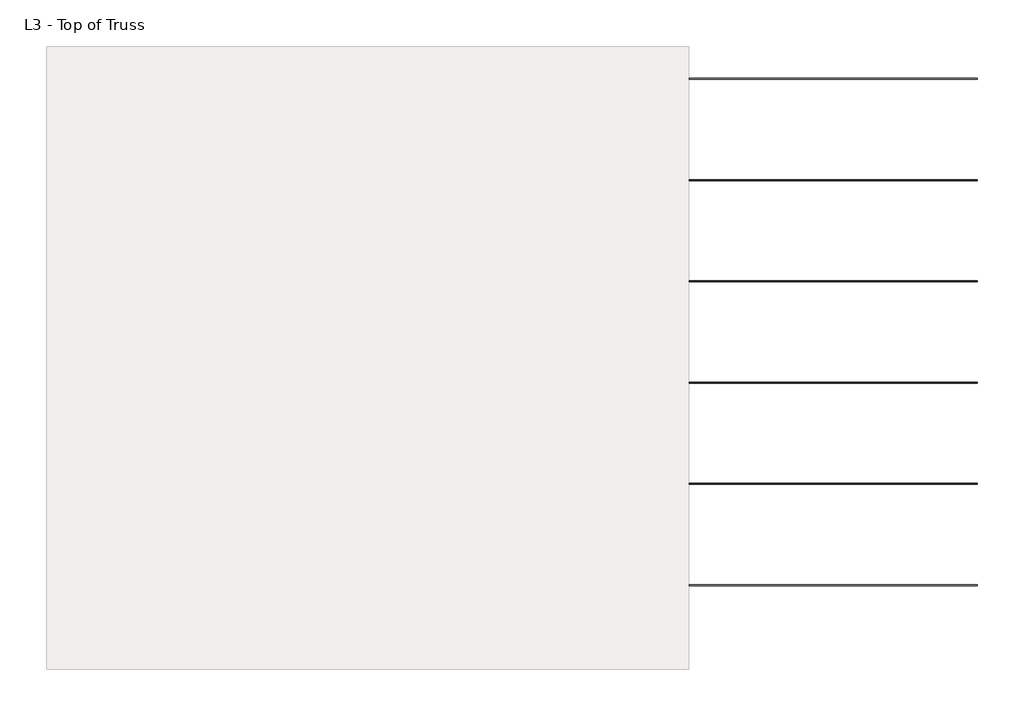
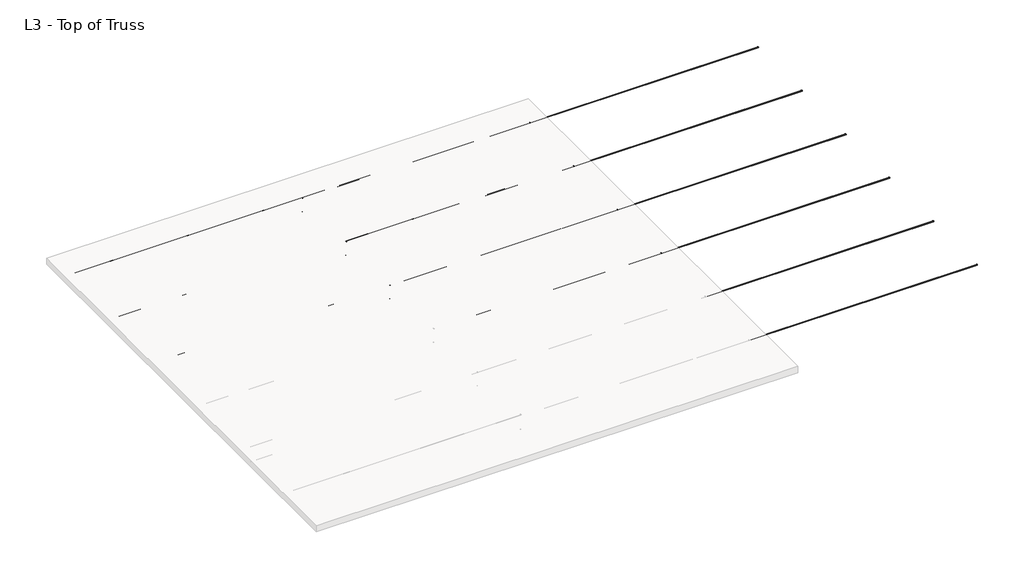
# One storey, part 2 of 2: 101 beams.
"""IFC4 building model written with IfcOpenShell, lengths in millimetres."""

import ifcopenshell
import ifcopenshell.guid

model = None  # the IFC model being written
_history = None  # IfcOwnerHistory: only IFC2X3 demands one
_inside = {}  # id of a spatial element -> (the spatial element, [elements in it])
_under = {}  # id of a project, library or spatial element -> (it, [spatial elements below it])
_declared = {}  # id of a project -> (the project, [libraries it declares])
_typed = {}  # id of a type object -> (the type object, [elements of that type])
_made_of = {}  # id of a material, layer set ... -> (it, [elements and type objects made of it])


def new_model(schema):
    """Start an empty IFC model of exactly this schema.

    Asked for "IFC4X3", IfcOpenShell would pick the latest addendum, in which some entities
    have other attributes; the version numbers below select the first issue.
    IFC2X3 requires an IfcOwnerHistory on every rooted entity: one is made here for all.
    """
    global model, _history
    if schema == "IFC4X3":
        model = ifcopenshell.file(schema_version=(4, 3, 0, 0))
    else:
        model = ifcopenshell.file(schema=schema)
    _inside.clear()
    _under.clear()
    _declared.clear()
    _typed.clear()
    _made_of.clear()
    _history = None
    if model.schema == "IFC2X3":
        org = make("IfcOrganization", Name="unknown")
        user = make(
            "IfcPersonAndOrganization",
            ThePerson=make("IfcPerson", FamilyName="unknown"),
            TheOrganization=org,
        )
        app = make(
            "IfcApplication",
            ApplicationDeveloper=org,
            Version="unknown",
            ApplicationFullName="unknown",
            ApplicationIdentifier="unknown",
        )
        _history = make(
            "IfcOwnerHistory",
            OwningUser=user,
            OwningApplication=app,
            ChangeAction="ADDED",
            CreationDate=0,
        )
    return model


def make(cls, **values):
    """One entity of the class cls with the attributes given. An attribute that is None is left unset."""
    return model.create_entity(
        cls, **{name: value for name, value in values.items() if value is not None}
    )


def rooted(cls, **values):
    """An entity with a GlobalId (a new one), such as an element, a storey or a relation."""
    return make(cls, GlobalId=ifcopenshell.guid.new(), OwnerHistory=_history, **values)


def si_unit(unit_type, name, prefix=None):
    """IfcSIUnit, for example si_unit("LENGTHUNIT", "METRE", prefix="MILLI")."""
    return make("IfcSIUnit", UnitType=unit_type, Prefix=prefix, Name=name)


def assignment(units):
    """IfcUnitAssignment: the units of a project."""
    return None if units is None else make("IfcUnitAssignment", Units=units)


def point(xyz):
    """IfcCartesianPoint."""
    return None if xyz is None else make("IfcCartesianPoint", Coordinates=xyz)


def direction(xyz):
    """IfcDirection."""
    return None if xyz is None else make("IfcDirection", DirectionRatios=xyz)


def frame(location, z_axis=None, x_axis=None):
    """IfcAxis2Placement3D, a coordinate frame: its origin and axes. An axis left out is left unset."""
    return make(
        "IfcAxis2Placement3D",
        Location=point(location),
        Axis=direction(z_axis),
        RefDirection=direction(x_axis),
    )


def frame_2d(location, x_axis=None):
    """IfcAxis2Placement2D, a coordinate frame in the plane: its origin and x axis."""
    return make(
        "IfcAxis2Placement2D", Location=point(location), RefDirection=direction(x_axis)
    )


def origin():
    """The frame at (0, 0, 0) with its axes left unset."""
    return frame((0.0, 0.0, 0.0))


def origin_2d():
    """The frame at (0, 0) in the plane with its x axis left unset."""
    return frame_2d((0.0, 0.0))


def place(relative_to, where):
    """IfcLocalPlacement: puts the frame where relative to a parent placement (None: the world)."""
    return make(
        "IfcLocalPlacement", PlacementRelTo=relative_to, RelativePlacement=where
    )


def context(
    kind, dimensions, precision=None, world=None, true_north=None, identifier=None
):
    """IfcGeometricRepresentationContext, for example the 3D "Model" context."""
    return make(
        "IfcGeometricRepresentationContext",
        ContextIdentifier=identifier,
        ContextType=kind,
        CoordinateSpaceDimension=dimensions,
        Precision=precision,
        WorldCoordinateSystem=world,
        TrueNorth=true_north,
    )


def project(units=None, contexts=None):
    """IfcProject with its units and contexts."""
    return rooted(
        "IfcProject",
        Name="project",
        RepresentationContexts=contexts,
        UnitsInContext=assignment(units),
    )


def spatial(cls, under=None, at=None, **own):
    """A site, building, storey or space (cls), placed at a placement, below another one or the project."""
    s = rooted(cls, ObjectPlacement=at, **own)
    if under is not None:
        _under.setdefault(under.id(), (under, []))[1].append(s)
    return s


def circle_curve(where, radius):
    """IfcCircle in the frame where."""
    return make("IfcCircle", Position=where, Radius=radius)


def trimmed(basis, trim1, trim2, sense, master):
    """IfcTrimmedCurve: the piece of a basis curve between two trims."""
    return make(
        "IfcTrimmedCurve",
        BasisCurve=basis,
        Trim1=trim1,
        Trim2=trim2,
        SenseAgreement=sense,
        MasterRepresentation=master,
    )


def segment(curve, same_sense, transition):
    """IfcCompositeCurveSegment."""
    return make(
        "IfcCompositeCurveSegment",
        Transition=transition,
        SameSense=same_sense,
        ParentCurve=curve,
    )


def composite_curve(segments, self_intersect=None):
    """IfcCompositeCurve: segments joined end to end."""
    return make("IfcCompositeCurve", Segments=segments, SelfIntersect=self_intersect)


def outline(outer, holes=None, kind="AREA"):
    """IfcArbitraryClosedProfileDef: a profile drawn as a closed curve; with holes, ...WithVoids."""
    if holes is None:
        return make("IfcArbitraryClosedProfileDef", ProfileType=kind, OuterCurve=outer)
    return make(
        "IfcArbitraryProfileDefWithVoids",
        ProfileType=kind,
        OuterCurve=outer,
        InnerCurves=holes,
    )


def extrude(swept, where, along, depth):
    """IfcExtrudedAreaSolid: the profile swept, set in the frame where, extruded along a direction by depth."""
    return make(
        "IfcExtrudedAreaSolid",
        SweptArea=swept,
        Position=where,
        ExtrudedDirection=direction(along),
        Depth=depth,
    )


def shape(context_of_items, identifier, shape_type, items):
    """IfcShapeRepresentation: the items that make up one representation, for example the "Body"."""
    return make(
        "IfcShapeRepresentation",
        ContextOfItems=context_of_items,
        RepresentationIdentifier=identifier,
        RepresentationType=shape_type,
        Items=items,
    )


def source(mapping_origin, context_of_items, identifier, shape_type, items):
    """IfcRepresentationMap: a shape defined once, which mapped items show again and again."""
    return make(
        "IfcRepresentationMap",
        MappingOrigin=mapping_origin,
        MappedRepresentation=shape(context_of_items, identifier, shape_type, items),
    )


def transform(
    local_origin,
    x_axis=None,
    y_axis=None,
    z_axis=None,
    scale=None,
    scale2=None,
    scale3=None,
    uniform=True,
):
    """IfcCartesianTransformationOperator3D, or its non-uniform kind. x_axis, y_axis, z_axis: its Axis1, 2, 3."""
    if uniform:
        return make(
            "IfcCartesianTransformationOperator3D",
            Axis1=direction(x_axis),
            Axis2=direction(y_axis),
            LocalOrigin=point(local_origin),
            Scale=scale,
            Axis3=direction(z_axis),
        )
    return make(
        "IfcCartesianTransformationOperator3DnonUniform",
        Axis1=direction(x_axis),
        Axis2=direction(y_axis),
        LocalOrigin=point(local_origin),
        Scale=scale,
        Axis3=direction(z_axis),
        Scale2=scale2,
        Scale3=scale3,
    )


def mapped(mapping_source, mapping_target):
    """IfcMappedItem: shows the shape of a source again, moved by a transform."""
    return make(
        "IfcMappedItem", MappingSource=mapping_source, MappingTarget=mapping_target
    )


def made_of(thing, what):
    """Note that an element or type object is made of a material, layer set ...; save() writes the relation."""
    if what is not None:
        _made_of.setdefault(what.id(), (what, []))[1].append(thing)
    return thing


def element(
    cls,
    number,
    at=None,
    inside=None,
    cuts=None,
    type_object=None,
    material=None,
    context=None,
    identifier="Body",
    shape_type=None,
    held_by="IfcProductDefinitionShape",
    body=None,
    shapes=None,
    **own,
):
    """One element of the class cls, such as IfcWall. Its Tag is "e" and its number.

    at: its placement. inside: the storey or other place that contains it. cuts: it is an
    opening in that element (IfcRelVoidsElement). A single representation is given by context,
    identifier, shape_type and body (its items); several are given by shapes. held_by: the class
    of the entity that holds the representations. save() writes the other relations.
    """
    e = rooted(cls, Tag="e%d" % number, ObjectPlacement=at, **own)
    if body is not None:
        shapes = [shape(context, identifier, shape_type, body)]
    if shapes is not None:
        e.Representation = make(held_by, Representations=shapes)
    if inside is not None:
        _inside.setdefault(inside.id(), (inside, []))[1].append(e)
    if cuts is not None:
        rooted(
            "IfcRelVoidsElement", RelatingBuildingElement=cuts, RelatedOpeningElement=e
        )
    if type_object is not None:
        _typed.setdefault(type_object.id(), (type_object, []))[1].append(e)
    return made_of(e, material)


def aggregate(whole, parts):
    """IfcRelAggregates: a whole, such as a stair, and the parts it consists of."""
    return rooted("IfcRelAggregates", RelatingObject=whole, RelatedObjects=parts)


def save(model, path):
    """Write the relations noted so far, then the file.

    IfcRelAggregates (storeys below a building ...), IfcRelContainedInSpatialStructure (elements
    in a storey), IfcRelDefinesByType, IfcRelAssociatesMaterial and IfcRelDeclares: one each for
    every whole, place, type object, material and project.
    """
    for whole, parts in _under.values():
        aggregate(whole, parts)
    for where, things in _inside.values():
        rooted(
            "IfcRelContainedInSpatialStructure",
            RelatedElements=things,
            RelatingStructure=where,
        )
    for kind, things in _typed.values():
        rooted("IfcRelDefinesByType", RelatedObjects=things, RelatingType=kind)
    for what, things in _made_of.values():
        rooted("IfcRelAssociatesMaterial", RelatedObjects=things, RelatingMaterial=what)
    for by, libraries in _declared.values():
        rooted("IfcRelDeclares", RelatingContext=by, RelatedDefinitions=libraries)
    model.write(path)


def circular_hollow_sections_chs60_3x5_c94bd862(model_context):
    return source(origin(), model_context, "Body", "SweptSolid", [
        extrude(outline(composite_curve([segment(trimmed(circle_curve(origin_2d(), 30.15), [point((-30.15, 0.0))], [point((30.15, 0.0))], False, "CARTESIAN"), True, "CONTINUOUS"), segment(trimmed(circle_curve(origin_2d(), 30.15), [point((30.15, 0.0))], [point((-30.15, 0.0))], False, "CARTESIAN"), True, "CONTINUOUS")], self_intersect=False), holes=[composite_curve([segment(trimmed(circle_curve(origin_2d(), 25.15), [point((25.15, 0.0))], [point((-25.15, 0.0))], True, "CARTESIAN"), True, "CONTINUOUS"), segment(trimmed(circle_curve(origin_2d(), 25.15), [point((-25.15, 0.0))], [point((25.15, 0.0))], True, "CARTESIAN"), True, "CONTINUOUS")], self_intersect=False)]), frame((-557.0, 0.0, 0.0), z_axis=(1.0, 0.0, 0.0), x_axis=(0.0, 1.0, 0.0)), (0.0, 0.0, 1.0), 1114.0),
    ])


def circular_hollow_sections_chs60_3x5_b8a643cb(model_context):
    return source(origin(), model_context, "Body", "SweptSolid", [
        extrude(outline(composite_curve([segment(trimmed(circle_curve(origin_2d(), 30.15), [point((-30.15, 0.0))], [point((30.15, 0.0))], False, "CARTESIAN"), True, "CONTINUOUS"), segment(trimmed(circle_curve(origin_2d(), 30.15), [point((30.15, 0.0))], [point((-30.15, 0.0))], False, "CARTESIAN"), True, "CONTINUOUS")], self_intersect=False), holes=[composite_curve([segment(trimmed(circle_curve(origin_2d(), 25.15), [point((25.15, 0.0))], [point((-25.15, 0.0))], True, "CARTESIAN"), True, "CONTINUOUS"), segment(trimmed(circle_curve(origin_2d(), 25.15), [point((-25.15, 0.0))], [point((25.15, 0.0))], True, "CARTESIAN"), True, "CONTINUOUS")], self_intersect=False)]), frame((-790.0, 0.0, 0.0), z_axis=(1.0, 0.0, 0.0), x_axis=(0.0, 1.0, 0.0)), (0.0, 0.0, 1.0), 1580.0),
    ])


def circular_hollow_sections_chs60_3x5_ee2473de(model_context):
    return source(origin(), model_context, "Body", "SweptSolid", [
        extrude(outline(composite_curve([segment(trimmed(circle_curve(origin_2d(), 30.15), [point((-30.15, 0.0))], [point((30.15, 0.0))], False, "CARTESIAN"), True, "CONTINUOUS"), segment(trimmed(circle_curve(origin_2d(), 30.15), [point((30.15, 0.0))], [point((-30.15, 0.0))], False, "CARTESIAN"), True, "CONTINUOUS")], self_intersect=False), holes=[composite_curve([segment(trimmed(circle_curve(origin_2d(), 25.15), [point((25.15, 0.0))], [point((-25.15, 0.0))], True, "CARTESIAN"), True, "CONTINUOUS"), segment(trimmed(circle_curve(origin_2d(), 25.15), [point((-25.15, 0.0))], [point((25.15, 0.0))], True, "CARTESIAN"), True, "CONTINUOUS")], self_intersect=False)]), frame((-9000.0, 0.0, 0.0), z_axis=(1.0, 0.0, 0.0), x_axis=(0.0, 1.0, 0.0)), (0.0, 0.0, 1.0), 18000.0),
    ])


def circular_hollow_sections_chs60_3x5_7809bf4e(model_context):
    return source(origin(), model_context, "Body", "SweptSolid", [
        extrude(outline(composite_curve([segment(trimmed(circle_curve(origin_2d(), 30.15), [point((-30.15, 0.0))], [point((30.15, 0.0))], False, "CARTESIAN"), True, "CONTINUOUS"), segment(trimmed(circle_curve(origin_2d(), 30.15), [point((30.15, 0.0))], [point((-30.15, 0.0))], False, "CARTESIAN"), True, "CONTINUOUS")], self_intersect=False), holes=[composite_curve([segment(trimmed(circle_curve(origin_2d(), 25.15), [point((25.15, 0.0))], [point((-25.15, 0.0))], True, "CARTESIAN"), True, "CONTINUOUS"), segment(trimmed(circle_curve(origin_2d(), 25.15), [point((-25.15, 0.0))], [point((25.15, 0.0))], True, "CARTESIAN"), True, "CONTINUOUS")], self_intersect=False)]), frame((-600.0, 0.0, 0.0), z_axis=(1.0, 0.0, 0.0), x_axis=(0.0, 1.0, 0.0)), (0.0, 0.0, 1.0), 1157.0),
    ])


model = new_model("IFC4")

# Units and contexts
model_context = context("Model", 3, world=origin())
ifc_project = project(units=[si_unit("LENGTHUNIT", "METRE", prefix="MILLI")], contexts=[model_context])

# Site, building, storey
site = spatial("IfcSite", under=ifc_project)
building = spatial("IfcBuilding", under=site)
storey = spatial("IfcBuildingStorey", under=building, Name="L3 - Top of Truss", Elevation=7800.0)

# Beams
placement = place(None, origin())
circular_hollow_sections_chs60_3x5_shape = circular_hollow_sections_chs60_3x5_c94bd862(model_context)
element("IfcBeam", 1, ObjectType="Circular Hollow Sections : CHS60.3x5", at=placement, inside=storey, context=model_context, shape_type="MappedRepresentation", body=[
    mapped(circular_hollow_sections_chs60_3x5_shape, transform((9574.7303686, 941.2380918, 7200.0), x_axis=(0.0, 0.0, 1.0), y_axis=(0.0, -1.0, 0.0), z_axis=(1.0, 0.0, 0.0))),
])
element("IfcBeam", 2, ObjectType="Circular Hollow Sections : CHS60.3x5", at=placement, inside=storey, context=model_context, shape_type="MappedRepresentation", body=[
    mapped(circular_hollow_sections_chs60_3x5_shape, transform((-5853.84106, 941.2380918, 7200.0), x_axis=(0.0, 0.0, 1.0), y_axis=(0.0, -1.0, 0.0), z_axis=(1.0, 0.0, 0.0))),
])
element("IfcBeam", 3, ObjectType="Circular Hollow Sections : CHS60.3x5", at=placement, inside=storey, context=model_context, shape_type="MappedRepresentation", body=[
    mapped(circular_hollow_sections_chs60_3x5_shape, transform((8289.0160829, 941.2380918, 7200.0), x_axis=(0.0, 0.0, 1.0), y_axis=(0.0, -1.0, 0.0), z_axis=(1.0, 0.0, 0.0))),
])
element("IfcBeam", 4, ObjectType="Circular Hollow Sections : CHS60.3x5", at=placement, inside=storey, context=model_context, shape_type="MappedRepresentation", body=[
    mapped(circular_hollow_sections_chs60_3x5_shape, transform((-4568.1267743, 941.2380918, 7200.0), x_axis=(0.0, 0.0, 1.0), y_axis=(0.0, -1.0, 0.0), z_axis=(1.0, 0.0, 0.0))),
])
element("IfcBeam", 5, ObjectType="Circular Hollow Sections : CHS60.3x5", at=placement, inside=storey, context=model_context, shape_type="MappedRepresentation", body=[
    mapped(circular_hollow_sections_chs60_3x5_shape, transform((7003.3017972, 941.2380918, 7200.0), x_axis=(0.0, 0.0, 1.0), y_axis=(0.0, -1.0, 0.0), z_axis=(1.0, 0.0, 0.0))),
])
element("IfcBeam", 6, ObjectType="Circular Hollow Sections : CHS60.3x5", at=placement, inside=storey, context=model_context, shape_type="MappedRepresentation", body=[
    mapped(circular_hollow_sections_chs60_3x5_shape, transform((-3282.4124885, 941.2380918, 7200.0), x_axis=(0.0, 0.0, 1.0), y_axis=(0.0, -1.0, 0.0), z_axis=(1.0, 0.0, 0.0))),
])
element("IfcBeam", 7, ObjectType="Circular Hollow Sections : CHS60.3x5", at=placement, inside=storey, context=model_context, shape_type="MappedRepresentation", body=[
    mapped(circular_hollow_sections_chs60_3x5_shape, transform((5717.5875115, 941.2380918, 7200.0), x_axis=(0.0, 0.0, 1.0), y_axis=(0.0, -1.0, 0.0), z_axis=(1.0, 0.0, 0.0))),
])
element("IfcBeam", 8, ObjectType="Circular Hollow Sections : CHS60.3x5", at=placement, inside=storey, context=model_context, shape_type="MappedRepresentation", body=[
    mapped(circular_hollow_sections_chs60_3x5_shape, transform((4431.8732257, 941.2380918, 7200.0), x_axis=(0.0, 0.0, 1.0), y_axis=(0.0, -1.0, 0.0), z_axis=(1.0, 0.0, 0.0))),
])
element("IfcBeam", 9, ObjectType="Circular Hollow Sections : CHS60.3x5", at=placement, inside=storey, context=model_context, shape_type="MappedRepresentation", body=[
    mapped(circular_hollow_sections_chs60_3x5_shape, transform((3146.15894, 941.2380918, 7200.0), x_axis=(0.0, 0.0, 1.0), y_axis=(0.0, -1.0, 0.0), z_axis=(1.0, 0.0, 0.0))),
])
element("IfcBeam", 10, ObjectType="Circular Hollow Sections : CHS60.3x5", at=placement, inside=storey, context=model_context, shape_type="MappedRepresentation", body=[
    mapped(circular_hollow_sections_chs60_3x5_shape, transform((-1996.6982028, 941.2380918, 7200.0), x_axis=(0.0, 0.0, 1.0), y_axis=(0.0, -1.0, 0.0), z_axis=(1.0, 0.0, 0.0))),
])
element("IfcBeam", 11, ObjectType="Circular Hollow Sections : CHS60.3x5", at=placement, inside=storey, context=model_context, shape_type="MappedRepresentation", body=[
    mapped(circular_hollow_sections_chs60_3x5_shape, transform((-710.9839171, 941.2380918, 7200.0), x_axis=(0.0, 0.0, 1.0), y_axis=(0.0, -1.0, 0.0), z_axis=(1.0, 0.0, 0.0))),
])
element("IfcBeam", 12, ObjectType="Circular Hollow Sections : CHS60.3x5", at=placement, inside=storey, context=model_context, shape_type="MappedRepresentation", body=[
    mapped(circular_hollow_sections_chs60_3x5_shape, transform((574.7303686, 941.2380918, 7200.0), x_axis=(0.0, 0.0, 1.0), y_axis=(0.0, -1.0, 0.0), z_axis=(1.0, 0.0, 0.0))),
])
element("IfcBeam", 13, ObjectType="Circular Hollow Sections : CHS60.3x5", at=placement, inside=storey, context=model_context, shape_type="MappedRepresentation", body=[
    mapped(circular_hollow_sections_chs60_3x5_shape, transform((1860.4446543, 941.2380918, 7200.0), x_axis=(0.0, 0.0, 1.0), y_axis=(0.0, -1.0, 0.0), z_axis=(1.0, 0.0, 0.0))),
])
element("IfcBeam", 14, ObjectType="Circular Hollow Sections : CHS60.3x5", at=placement, inside=storey, context=model_context, shape_type="MappedRepresentation", body=[
    mapped(circular_hollow_sections_chs60_3x5_shape, transform((9574.7303686, 6941.2380918, 7200.0), x_axis=(0.0, 0.0, 1.0), y_axis=(0.0, -1.0, 0.0), z_axis=(1.0, 0.0, 0.0))),
])
element("IfcBeam", 15, ObjectType="Circular Hollow Sections : CHS60.3x5", at=placement, inside=storey, context=model_context, shape_type="MappedRepresentation", body=[
    mapped(circular_hollow_sections_chs60_3x5_shape, transform((-5853.84106, 6941.2380918, 7200.0), x_axis=(0.0, 0.0, 1.0), y_axis=(0.0, -1.0, 0.0), z_axis=(1.0, 0.0, 0.0))),
])
element("IfcBeam", 16, ObjectType="Circular Hollow Sections : CHS60.3x5", at=placement, inside=storey, context=model_context, shape_type="MappedRepresentation", body=[
    mapped(circular_hollow_sections_chs60_3x5_shape, transform((8289.0160829, 6941.2380918, 7200.0), x_axis=(0.0, 0.0, 1.0), y_axis=(0.0, -1.0, 0.0), z_axis=(1.0, 0.0, 0.0))),
])
element("IfcBeam", 17, ObjectType="Circular Hollow Sections : CHS60.3x5", at=placement, inside=storey, context=model_context, shape_type="MappedRepresentation", body=[
    mapped(circular_hollow_sections_chs60_3x5_shape, transform((-4568.1267743, 6941.2380918, 7200.0), x_axis=(0.0, 0.0, 1.0), y_axis=(0.0, -1.0, 0.0), z_axis=(1.0, 0.0, 0.0))),
])
element("IfcBeam", 18, ObjectType="Circular Hollow Sections : CHS60.3x5", at=placement, inside=storey, context=model_context, shape_type="MappedRepresentation", body=[
    mapped(circular_hollow_sections_chs60_3x5_shape, transform((7003.3017972, 6941.2380918, 7200.0), x_axis=(0.0, 0.0, 1.0), y_axis=(0.0, -1.0, 0.0), z_axis=(1.0, 0.0, 0.0))),
])
element("IfcBeam", 19, ObjectType="Circular Hollow Sections : CHS60.3x5", at=placement, inside=storey, context=model_context, shape_type="MappedRepresentation", body=[
    mapped(circular_hollow_sections_chs60_3x5_shape, transform((-3282.4124885, 6941.2380918, 7200.0), x_axis=(0.0, 0.0, 1.0), y_axis=(0.0, -1.0, 0.0), z_axis=(1.0, 0.0, 0.0))),
])
element("IfcBeam", 20, ObjectType="Circular Hollow Sections : CHS60.3x5", at=placement, inside=storey, context=model_context, shape_type="MappedRepresentation", body=[
    mapped(circular_hollow_sections_chs60_3x5_shape, transform((5717.5875115, 6941.2380918, 7200.0), x_axis=(0.0, 0.0, 1.0), y_axis=(0.0, -1.0, 0.0), z_axis=(1.0, 0.0, 0.0))),
])
element("IfcBeam", 21, ObjectType="Circular Hollow Sections : CHS60.3x5", at=placement, inside=storey, context=model_context, shape_type="MappedRepresentation", body=[
    mapped(circular_hollow_sections_chs60_3x5_shape, transform((4431.8732257, 6941.2380918, 7200.0), x_axis=(0.0, 0.0, 1.0), y_axis=(0.0, -1.0, 0.0), z_axis=(1.0, 0.0, 0.0))),
])
element("IfcBeam", 22, ObjectType="Circular Hollow Sections : CHS60.3x5", at=placement, inside=storey, context=model_context, shape_type="MappedRepresentation", body=[
    mapped(circular_hollow_sections_chs60_3x5_shape, transform((3146.15894, 6941.2380918, 7200.0), x_axis=(0.0, 0.0, 1.0), y_axis=(0.0, -1.0, 0.0), z_axis=(1.0, 0.0, 0.0))),
])
element("IfcBeam", 23, ObjectType="Circular Hollow Sections : CHS60.3x5", at=placement, inside=storey, context=model_context, shape_type="MappedRepresentation", body=[
    mapped(circular_hollow_sections_chs60_3x5_shape, transform((-1996.6982028, 6941.2380918, 7200.0), x_axis=(0.0, 0.0, 1.0), y_axis=(0.0, -1.0, 0.0), z_axis=(1.0, 0.0, 0.0))),
])
element("IfcBeam", 24, ObjectType="Circular Hollow Sections : CHS60.3x5", at=placement, inside=storey, context=model_context, shape_type="MappedRepresentation", body=[
    mapped(circular_hollow_sections_chs60_3x5_shape, transform((-710.9839171, 6941.2380918, 7200.0), x_axis=(0.0, 0.0, 1.0), y_axis=(0.0, -1.0, 0.0), z_axis=(1.0, 0.0, 0.0))),
])
element("IfcBeam", 25, ObjectType="Circular Hollow Sections : CHS60.3x5", at=placement, inside=storey, context=model_context, shape_type="MappedRepresentation", body=[
    mapped(circular_hollow_sections_chs60_3x5_shape, transform((574.7303686, 6941.2380918, 7200.0), x_axis=(0.0, 0.0, 1.0), y_axis=(0.0, -1.0, 0.0), z_axis=(1.0, 0.0, 0.0))),
])
element("IfcBeam", 26, ObjectType="Circular Hollow Sections : CHS60.3x5", at=placement, inside=storey, context=model_context, shape_type="MappedRepresentation", body=[
    mapped(circular_hollow_sections_chs60_3x5_shape, transform((1860.4446543, 6941.2380918, 7200.0), x_axis=(0.0, 0.0, 1.0), y_axis=(0.0, -1.0, 0.0), z_axis=(1.0, 0.0, 0.0))),
])
element("IfcBeam", 27, ObjectType="Circular Hollow Sections : CHS60.3x5", at=placement, inside=storey, context=model_context, shape_type="MappedRepresentation", body=[
    mapped(circular_hollow_sections_chs60_3x5_shape, transform((9574.7303686, -5058.7619082, 7200.0), x_axis=(0.0, 0.0, 1.0), y_axis=(0.0, -1.0, 0.0), z_axis=(1.0, 0.0, 0.0))),
])
element("IfcBeam", 28, ObjectType="Circular Hollow Sections : CHS60.3x5", at=placement, inside=storey, context=model_context, shape_type="MappedRepresentation", body=[
    mapped(circular_hollow_sections_chs60_3x5_shape, transform((8289.0160829, -5058.7619082, 7200.0), x_axis=(0.0, 0.0, 1.0), y_axis=(0.0, -1.0, 0.0), z_axis=(1.0, 0.0, 0.0))),
])
element("IfcBeam", 29, ObjectType="Circular Hollow Sections : CHS60.3x5", at=placement, inside=storey, context=model_context, shape_type="MappedRepresentation", body=[
    mapped(circular_hollow_sections_chs60_3x5_shape, transform((7003.3017972, -5058.7619082, 7200.0), x_axis=(0.0, 0.0, 1.0), y_axis=(0.0, -1.0, 0.0), z_axis=(1.0, 0.0, 0.0))),
])
element("IfcBeam", 30, ObjectType="Circular Hollow Sections : CHS60.3x5", at=placement, inside=storey, context=model_context, shape_type="MappedRepresentation", body=[
    mapped(circular_hollow_sections_chs60_3x5_shape, transform((5717.5875115, -5058.7619082, 7200.0), x_axis=(0.0, 0.0, 1.0), y_axis=(0.0, -1.0, 0.0), z_axis=(1.0, 0.0, 0.0))),
])
element("IfcBeam", 31, ObjectType="Circular Hollow Sections : CHS60.3x5", at=placement, inside=storey, context=model_context, shape_type="MappedRepresentation", body=[
    mapped(circular_hollow_sections_chs60_3x5_shape, transform((4431.8732257, -5058.7619082, 7200.0), x_axis=(0.0, 0.0, 1.0), y_axis=(0.0, -1.0, 0.0), z_axis=(1.0, 0.0, 0.0))),
])
element("IfcBeam", 32, ObjectType="Circular Hollow Sections : CHS60.3x5", at=placement, inside=storey, context=model_context, shape_type="MappedRepresentation", body=[
    mapped(circular_hollow_sections_chs60_3x5_shape, transform((3146.15894, -5058.7619082, 7200.0), x_axis=(0.0, 0.0, 1.0), y_axis=(0.0, -1.0, 0.0), z_axis=(1.0, 0.0, 0.0))),
])
element("IfcBeam", 33, ObjectType="Circular Hollow Sections : CHS60.3x5", at=placement, inside=storey, context=model_context, shape_type="MappedRepresentation", body=[
    mapped(circular_hollow_sections_chs60_3x5_shape, transform((574.7303686, -5058.7619082, 7200.0), x_axis=(0.0, 0.0, 1.0), y_axis=(0.0, -1.0, 0.0), z_axis=(1.0, 0.0, 0.0))),
])
element("IfcBeam", 34, ObjectType="Circular Hollow Sections : CHS60.3x5", at=placement, inside=storey, context=model_context, shape_type="MappedRepresentation", body=[
    mapped(circular_hollow_sections_chs60_3x5_shape, transform((1860.4446543, -5058.7619082, 7200.0), x_axis=(0.0, 0.0, 1.0), y_axis=(0.0, -1.0, 0.0), z_axis=(1.0, 0.0, 0.0))),
])
element("IfcBeam", 35, ObjectType="Circular Hollow Sections : CHS60.3x5", at=placement, inside=storey, context=model_context, shape_type="MappedRepresentation", body=[
    mapped(circular_hollow_sections_chs60_3x5_shape, transform((9574.7303686, -11058.7619082, 7200.0), x_axis=(0.0, 0.0, 1.0), y_axis=(0.0, -1.0, 0.0), z_axis=(1.0, 0.0, 0.0))),
])
element("IfcBeam", 36, ObjectType="Circular Hollow Sections : CHS60.3x5", at=placement, inside=storey, context=model_context, shape_type="MappedRepresentation", body=[
    mapped(circular_hollow_sections_chs60_3x5_shape, transform((8289.0160829, -11058.7619082, 7200.0), x_axis=(0.0, 0.0, 1.0), y_axis=(0.0, -1.0, 0.0), z_axis=(1.0, 0.0, 0.0))),
])
element("IfcBeam", 37, ObjectType="Circular Hollow Sections : CHS60.3x5", at=placement, inside=storey, context=model_context, shape_type="MappedRepresentation", body=[
    mapped(circular_hollow_sections_chs60_3x5_shape, transform((7003.3017972, -11058.7619082, 7200.0), x_axis=(0.0, 0.0, 1.0), y_axis=(0.0, -1.0, 0.0), z_axis=(1.0, 0.0, 0.0))),
])
circular_hollow_sections_chs60_3x5_2_shape = circular_hollow_sections_chs60_3x5_b8a643cb(model_context)
element("IfcBeam", 38, ObjectType="Circular Hollow Sections : CHS60.3x5", at=placement, inside=storey, context=model_context, shape_type="MappedRepresentation", body=[
    mapped(circular_hollow_sections_chs60_3x5_2_shape, transform((8931.8732257, 941.2380918, 7200.0), x_axis=(0.7310552682428691, 0.0, 0.6823182503600111), y_axis=(0.0, -1.0, 0.0), z_axis=(0.6823182503600111, 0.0, -0.7310552682428691))),
])
element("IfcBeam", 39, ObjectType="Circular Hollow Sections : CHS60.3x5", at=placement, inside=storey, context=model_context, shape_type="MappedRepresentation", body=[
    mapped(circular_hollow_sections_chs60_3x5_2_shape, transform((-5210.9839171, 941.2380918, 7200.0), x_axis=(0.7310552682428689, 0.0, -0.6823182503600113), y_axis=(0.0, -1.0, 0.0), z_axis=(-0.6823182503600113, 0.0, -0.7310552682428689))),
])
element("IfcBeam", 40, ObjectType="Circular Hollow Sections : CHS60.3x5", at=placement, inside=storey, context=model_context, shape_type="MappedRepresentation", body=[
    mapped(circular_hollow_sections_chs60_3x5_2_shape, transform((7646.15894, 941.2380918, 7200.0), x_axis=(0.7310552682428691, 0.0, 0.6823182503600111), y_axis=(0.0, -1.0, 0.0), z_axis=(0.6823182503600111, 0.0, -0.7310552682428691))),
])
element("IfcBeam", 41, ObjectType="Circular Hollow Sections : CHS60.3x5", at=placement, inside=storey, context=model_context, shape_type="MappedRepresentation", body=[
    mapped(circular_hollow_sections_chs60_3x5_2_shape, transform((-3925.2696314, 941.2380918, 7200.0), x_axis=(0.7310552682428689, 0.0, -0.6823182503600113), y_axis=(0.0, -1.0, 0.0), z_axis=(-0.6823182503600113, 0.0, -0.7310552682428689))),
])
element("IfcBeam", 42, ObjectType="Circular Hollow Sections : CHS60.3x5", at=placement, inside=storey, context=model_context, shape_type="MappedRepresentation", body=[
    mapped(circular_hollow_sections_chs60_3x5_2_shape, transform((6360.4446543, 941.2380918, 7200.0), x_axis=(0.7310552682428691, 0.0, 0.6823182503600111), y_axis=(0.0, -1.0, 0.0), z_axis=(0.6823182503600111, 0.0, -0.7310552682428691))),
])
element("IfcBeam", 43, ObjectType="Circular Hollow Sections : CHS60.3x5", at=placement, inside=storey, context=model_context, shape_type="MappedRepresentation", body=[
    mapped(circular_hollow_sections_chs60_3x5_2_shape, transform((-2639.5553457, 941.2380918, 7200.0), x_axis=(0.7310552682428689, 0.0, -0.6823182503600113), y_axis=(0.0, -1.0, 0.0), z_axis=(-0.6823182503600113, 0.0, -0.7310552682428689))),
])
element("IfcBeam", 44, ObjectType="Circular Hollow Sections : CHS60.3x5", at=placement, inside=storey, context=model_context, shape_type="MappedRepresentation", body=[
    mapped(circular_hollow_sections_chs60_3x5_2_shape, transform((5074.7303686, 941.2380918, 7200.0), x_axis=(0.7310552682428691, 0.0, 0.6823182503600111), y_axis=(0.0, -1.0, 0.0), z_axis=(0.6823182503600111, 0.0, -0.7310552682428691))),
])
element("IfcBeam", 45, ObjectType="Circular Hollow Sections : CHS60.3x5", at=placement, inside=storey, context=model_context, shape_type="MappedRepresentation", body=[
    mapped(circular_hollow_sections_chs60_3x5_2_shape, transform((3789.0160829, 941.2380918, 7200.0), x_axis=(0.7310552682428691, 0.0, 0.6823182503600111), y_axis=(0.0, -1.0, 0.0), z_axis=(0.6823182503600111, 0.0, -0.7310552682428691))),
])
element("IfcBeam", 46, ObjectType="Circular Hollow Sections : CHS60.3x5", at=placement, inside=storey, context=model_context, shape_type="MappedRepresentation", body=[
    mapped(circular_hollow_sections_chs60_3x5_2_shape, transform((10217.5875115, 941.2380918, 7200.0), x_axis=(0.7310552682428691, 0.0, 0.6823182503600111), y_axis=(0.0, -1.0, 0.0), z_axis=(0.6823182503600111, 0.0, -0.7310552682428691))),
])
element("IfcBeam", 47, ObjectType="Circular Hollow Sections : CHS60.3x5", at=placement, inside=storey, context=model_context, shape_type="MappedRepresentation", body=[
    mapped(circular_hollow_sections_chs60_3x5_2_shape, transform((2503.3017972, 941.2380918, 7200.0), x_axis=(0.7310552682428691, 0.0, 0.682318250360011), y_axis=(0.0, -1.0, 0.0), z_axis=(0.682318250360011, 0.0, -0.7310552682428691))),
])
element("IfcBeam", 48, ObjectType="Circular Hollow Sections : CHS60.3x5", at=placement, inside=storey, context=model_context, shape_type="MappedRepresentation", body=[
    mapped(circular_hollow_sections_chs60_3x5_2_shape, transform((-1353.84106, 941.2380918, 7200.0), x_axis=(0.7310552682428689, 0.0, -0.6823182503600113), y_axis=(0.0, -1.0, 0.0), z_axis=(-0.6823182503600113, 0.0, -0.7310552682428689))),
])
element("IfcBeam", 49, ObjectType="Circular Hollow Sections : CHS60.3x5", at=placement, inside=storey, context=model_context, shape_type="MappedRepresentation", body=[
    mapped(circular_hollow_sections_chs60_3x5_2_shape, transform((-68.1267743, 941.2380918, 7200.0), x_axis=(0.7310552682428689, 0.0, -0.6823182503600113), y_axis=(0.0, -1.0, 0.0), z_axis=(-0.6823182503600113, 0.0, -0.7310552682428689))),
])
element("IfcBeam", 50, ObjectType="Circular Hollow Sections : CHS60.3x5", at=placement, inside=storey, context=model_context, shape_type="MappedRepresentation", body=[
    mapped(circular_hollow_sections_chs60_3x5_2_shape, transform((-6496.6982028, 941.2380918, 7200.0), x_axis=(0.7310552682428688, 0.0, -0.6823182503600115), y_axis=(0.0, -1.0, 0.0), z_axis=(-0.6823182503600115, 0.0, -0.7310552682428688))),
])
element("IfcBeam", 51, ObjectType="Circular Hollow Sections : CHS60.3x5", at=placement, inside=storey, context=model_context, shape_type="MappedRepresentation", body=[
    mapped(circular_hollow_sections_chs60_3x5_2_shape, transform((1217.5875115, 941.2380918, 7200.0), x_axis=(0.7310552682428689, 0.0, -0.6823182503600113), y_axis=(0.0, -1.0, 0.0), z_axis=(-0.6823182503600113, 0.0, -0.7310552682428689))),
])
element("IfcBeam", 52, ObjectType="Circular Hollow Sections : CHS60.3x5", at=placement, inside=storey, context=model_context, shape_type="MappedRepresentation", body=[
    mapped(circular_hollow_sections_chs60_3x5_2_shape, transform((8931.8732257, 6941.2380918, 7200.0), x_axis=(0.7310552682428691, 0.0, 0.6823182503600111), y_axis=(0.0, -1.0, 0.0), z_axis=(0.6823182503600111, 0.0, -0.7310552682428691))),
])
element("IfcBeam", 53, ObjectType="Circular Hollow Sections : CHS60.3x5", at=placement, inside=storey, context=model_context, shape_type="MappedRepresentation", body=[
    mapped(circular_hollow_sections_chs60_3x5_2_shape, transform((-5210.9839171, 6941.2380918, 7200.0), x_axis=(0.7310552682428689, 0.0, -0.6823182503600113), y_axis=(0.0, -1.0, 0.0), z_axis=(-0.6823182503600113, 0.0, -0.7310552682428689))),
])
element("IfcBeam", 54, ObjectType="Circular Hollow Sections : CHS60.3x5", at=placement, inside=storey, context=model_context, shape_type="MappedRepresentation", body=[
    mapped(circular_hollow_sections_chs60_3x5_2_shape, transform((7646.15894, 6941.2380918, 7200.0), x_axis=(0.7310552682428691, 0.0, 0.6823182503600111), y_axis=(0.0, -1.0, 0.0), z_axis=(0.6823182503600111, 0.0, -0.7310552682428691))),
])
element("IfcBeam", 55, ObjectType="Circular Hollow Sections : CHS60.3x5", at=placement, inside=storey, context=model_context, shape_type="MappedRepresentation", body=[
    mapped(circular_hollow_sections_chs60_3x5_2_shape, transform((-3925.2696314, 6941.2380918, 7200.0), x_axis=(0.7310552682428689, 0.0, -0.6823182503600113), y_axis=(0.0, -1.0, 0.0), z_axis=(-0.6823182503600113, 0.0, -0.7310552682428689))),
])
element("IfcBeam", 56, ObjectType="Circular Hollow Sections : CHS60.3x5", at=placement, inside=storey, context=model_context, shape_type="MappedRepresentation", body=[
    mapped(circular_hollow_sections_chs60_3x5_2_shape, transform((6360.4446543, 6941.2380918, 7200.0), x_axis=(0.7310552682428691, 0.0, 0.6823182503600111), y_axis=(0.0, -1.0, 0.0), z_axis=(0.6823182503600111, 0.0, -0.7310552682428691))),
])
element("IfcBeam", 57, ObjectType="Circular Hollow Sections : CHS60.3x5", at=placement, inside=storey, context=model_context, shape_type="MappedRepresentation", body=[
    mapped(circular_hollow_sections_chs60_3x5_2_shape, transform((-2639.5553457, 6941.2380918, 7200.0), x_axis=(0.7310552682428689, 0.0, -0.6823182503600113), y_axis=(0.0, -1.0, 0.0), z_axis=(-0.6823182503600113, 0.0, -0.7310552682428689))),
])
element("IfcBeam", 58, ObjectType="Circular Hollow Sections : CHS60.3x5", at=placement, inside=storey, context=model_context, shape_type="MappedRepresentation", body=[
    mapped(circular_hollow_sections_chs60_3x5_2_shape, transform((5074.7303686, 6941.2380918, 7200.0), x_axis=(0.7310552682428691, 0.0, 0.6823182503600111), y_axis=(0.0, -1.0, 0.0), z_axis=(0.6823182503600111, 0.0, -0.7310552682428691))),
])
element("IfcBeam", 59, ObjectType="Circular Hollow Sections : CHS60.3x5", at=placement, inside=storey, context=model_context, shape_type="MappedRepresentation", body=[
    mapped(circular_hollow_sections_chs60_3x5_2_shape, transform((3789.0160829, 6941.2380918, 7200.0), x_axis=(0.7310552682428691, 0.0, 0.6823182503600111), y_axis=(0.0, -1.0, 0.0), z_axis=(0.6823182503600111, 0.0, -0.7310552682428691))),
])
element("IfcBeam", 60, ObjectType="Circular Hollow Sections : CHS60.3x5", at=placement, inside=storey, context=model_context, shape_type="MappedRepresentation", body=[
    mapped(circular_hollow_sections_chs60_3x5_2_shape, transform((10217.5875115, 6941.2380918, 7200.0), x_axis=(0.7310552682428691, 0.0, 0.6823182503600111), y_axis=(0.0, -1.0, 0.0), z_axis=(0.6823182503600111, 0.0, -0.7310552682428691))),
])
element("IfcBeam", 61, ObjectType="Circular Hollow Sections : CHS60.3x5", at=placement, inside=storey, context=model_context, shape_type="MappedRepresentation", body=[
    mapped(circular_hollow_sections_chs60_3x5_2_shape, transform((2503.3017972, 6941.2380918, 7200.0), x_axis=(0.7310552682428691, 0.0, 0.682318250360011), y_axis=(0.0, -1.0, 0.0), z_axis=(0.682318250360011, 0.0, -0.7310552682428691))),
])
element("IfcBeam", 62, ObjectType="Circular Hollow Sections : CHS60.3x5", at=placement, inside=storey, context=model_context, shape_type="MappedRepresentation", body=[
    mapped(circular_hollow_sections_chs60_3x5_2_shape, transform((-1353.84106, 6941.2380918, 7200.0), x_axis=(0.7310552682428689, 0.0, -0.6823182503600113), y_axis=(0.0, -1.0, 0.0), z_axis=(-0.6823182503600113, 0.0, -0.7310552682428689))),
])
element("IfcBeam", 63, ObjectType="Circular Hollow Sections : CHS60.3x5", at=placement, inside=storey, context=model_context, shape_type="MappedRepresentation", body=[
    mapped(circular_hollow_sections_chs60_3x5_2_shape, transform((-68.1267743, 6941.2380918, 7200.0), x_axis=(0.7310552682428689, 0.0, -0.6823182503600113), y_axis=(0.0, -1.0, 0.0), z_axis=(-0.6823182503600113, 0.0, -0.7310552682428689))),
])
element("IfcBeam", 64, ObjectType="Circular Hollow Sections : CHS60.3x5", at=placement, inside=storey, context=model_context, shape_type="MappedRepresentation", body=[
    mapped(circular_hollow_sections_chs60_3x5_2_shape, transform((-6496.6982028, 6941.2380918, 7200.0), x_axis=(0.7310552682428691, 0.0, -0.6823182503600111), y_axis=(0.0, -1.0, 0.0), z_axis=(-0.6823182503600111, 0.0, -0.7310552682428691))),
])
element("IfcBeam", 65, ObjectType="Circular Hollow Sections : CHS60.3x5", at=placement, inside=storey, context=model_context, shape_type="MappedRepresentation", body=[
    mapped(circular_hollow_sections_chs60_3x5_2_shape, transform((1217.5875115, 6941.2380918, 7200.0), x_axis=(0.7310552682428689, 0.0, -0.6823182503600113), y_axis=(0.0, -1.0, 0.0), z_axis=(-0.6823182503600113, 0.0, -0.7310552682428689))),
])
element("IfcBeam", 66, ObjectType="Circular Hollow Sections : CHS60.3x5", at=placement, inside=storey, context=model_context, shape_type="MappedRepresentation", body=[
    mapped(circular_hollow_sections_chs60_3x5_2_shape, transform((8931.8732257, -5058.7619082, 7200.0), x_axis=(0.7310552682428691, 0.0, 0.6823182503600111), y_axis=(0.0, -1.0, 0.0), z_axis=(0.6823182503600111, 0.0, -0.7310552682428691))),
])
element("IfcBeam", 67, ObjectType="Circular Hollow Sections : CHS60.3x5", at=placement, inside=storey, context=model_context, shape_type="MappedRepresentation", body=[
    mapped(circular_hollow_sections_chs60_3x5_2_shape, transform((7646.15894, -5058.7619082, 7200.0), x_axis=(0.7310552682428691, 0.0, 0.6823182503600111), y_axis=(0.0, -1.0, 0.0), z_axis=(0.6823182503600111, 0.0, -0.7310552682428691))),
])
element("IfcBeam", 68, ObjectType="Circular Hollow Sections : CHS60.3x5", at=placement, inside=storey, context=model_context, shape_type="MappedRepresentation", body=[
    mapped(circular_hollow_sections_chs60_3x5_2_shape, transform((6360.4446543, -5058.7619082, 7200.0), x_axis=(0.7310552682428691, 0.0, 0.6823182503600111), y_axis=(0.0, -1.0, 0.0), z_axis=(0.6823182503600111, 0.0, -0.7310552682428691))),
])
element("IfcBeam", 69, ObjectType="Circular Hollow Sections : CHS60.3x5", at=placement, inside=storey, context=model_context, shape_type="MappedRepresentation", body=[
    mapped(circular_hollow_sections_chs60_3x5_2_shape, transform((5074.7303686, -5058.7619082, 7200.0), x_axis=(0.7310552682428691, 0.0, 0.6823182503600111), y_axis=(0.0, -1.0, 0.0), z_axis=(0.6823182503600111, 0.0, -0.7310552682428691))),
])
element("IfcBeam", 70, ObjectType="Circular Hollow Sections : CHS60.3x5", at=placement, inside=storey, context=model_context, shape_type="MappedRepresentation", body=[
    mapped(circular_hollow_sections_chs60_3x5_2_shape, transform((3789.0160829, -5058.7619082, 7200.0), x_axis=(0.7310552682428691, 0.0, 0.6823182503600111), y_axis=(0.0, -1.0, 0.0), z_axis=(0.6823182503600111, 0.0, -0.7310552682428691))),
])
element("IfcBeam", 71, ObjectType="Circular Hollow Sections : CHS60.3x5", at=placement, inside=storey, context=model_context, shape_type="MappedRepresentation", body=[
    mapped(circular_hollow_sections_chs60_3x5_2_shape, transform((10217.5875115, -5058.7619082, 7200.0), x_axis=(0.7310552682428691, 0.0, 0.6823182503600111), y_axis=(0.0, -1.0, 0.0), z_axis=(0.6823182503600111, 0.0, -0.7310552682428691))),
])
element("IfcBeam", 72, ObjectType="Circular Hollow Sections : CHS60.3x5", at=placement, inside=storey, context=model_context, shape_type="MappedRepresentation", body=[
    mapped(circular_hollow_sections_chs60_3x5_2_shape, transform((2503.3017972, -5058.7619082, 7200.0), x_axis=(0.7310552682428691, 0.0, 0.682318250360011), y_axis=(0.0, -1.0, 0.0), z_axis=(0.682318250360011, 0.0, -0.7310552682428691))),
])
element("IfcBeam", 73, ObjectType="Circular Hollow Sections : CHS60.3x5", at=placement, inside=storey, context=model_context, shape_type="MappedRepresentation", body=[
    mapped(circular_hollow_sections_chs60_3x5_2_shape, transform((1217.5875115, -5058.7619082, 7200.0), x_axis=(0.7310552682428689, 0.0, -0.6823182503600113), y_axis=(0.0, -1.0, 0.0), z_axis=(-0.6823182503600113, 0.0, -0.7310552682428689))),
])
element("IfcBeam", 74, ObjectType="Circular Hollow Sections : CHS60.3x5", at=placement, inside=storey, context=model_context, shape_type="MappedRepresentation", body=[
    mapped(circular_hollow_sections_chs60_3x5_2_shape, transform((8931.8732257, -11058.7619082, 7200.0), x_axis=(0.7310552682428691, 0.0, 0.6823182503600111), y_axis=(0.0, -1.0, 0.0), z_axis=(0.6823182503600111, 0.0, -0.7310552682428691))),
])
element("IfcBeam", 75, ObjectType="Circular Hollow Sections : CHS60.3x5", at=placement, inside=storey, context=model_context, shape_type="MappedRepresentation", body=[
    mapped(circular_hollow_sections_chs60_3x5_2_shape, transform((7646.15894, -11058.7619082, 7200.0), x_axis=(0.7310552682428691, 0.0, 0.6823182503600111), y_axis=(0.0, -1.0, 0.0), z_axis=(0.6823182503600111, 0.0, -0.7310552682428691))),
])
element("IfcBeam", 76, ObjectType="Circular Hollow Sections : CHS60.3x5", at=placement, inside=storey, context=model_context, shape_type="MappedRepresentation", body=[
    mapped(circular_hollow_sections_chs60_3x5_2_shape, transform((6360.4446543, -11058.7619082, 7200.0), x_axis=(0.7310552682428691, 0.0, 0.6823182503600111), y_axis=(0.0, -1.0, 0.0), z_axis=(0.6823182503600111, 0.0, -0.7310552682428691))),
])
element("IfcBeam", 77, ObjectType="Circular Hollow Sections : CHS60.3x5", at=placement, inside=storey, context=model_context, shape_type="MappedRepresentation", body=[
    mapped(circular_hollow_sections_chs60_3x5_2_shape, transform((5074.7303686, -11058.7619082, 7200.0), x_axis=(0.7310552682428691, 0.0, 0.6823182503600111), y_axis=(0.0, -1.0, 0.0), z_axis=(0.6823182503600111, 0.0, -0.7310552682428691))),
])
element("IfcBeam", 78, ObjectType="Circular Hollow Sections : CHS60.3x5", at=placement, inside=storey, context=model_context, shape_type="MappedRepresentation", body=[
    mapped(circular_hollow_sections_chs60_3x5_2_shape, transform((10217.5875115, -11058.7619082, 7200.0), x_axis=(0.7310552682428691, 0.0, 0.6823182503600111), y_axis=(0.0, -1.0, 0.0), z_axis=(0.6823182503600111, 0.0, -0.7310552682428691))),
])
circular_hollow_sections_chs60_3x5_3_shape = circular_hollow_sections_chs60_3x5_ee2473de(model_context)
element("IfcBeam", 79, ObjectType="Circular Hollow Sections : CHS60.3x5", at=placement, inside=storey, context=model_context, shape_type="MappedRepresentation", body=[
    mapped(circular_hollow_sections_chs60_3x5_3_shape, transform((1860.4446543, 941.2380918, 6600.0), x_axis=(1.0, 0.0, 0.0), y_axis=(0.0, 1.0, 0.0), z_axis=(0.0, 0.0, 1.0))),
])
element("IfcBeam", 80, ObjectType="Circular Hollow Sections : CHS60.3x5", at=placement, inside=storey, context=model_context, shape_type="MappedRepresentation", body=[
    mapped(circular_hollow_sections_chs60_3x5_3_shape, transform((1860.4446543, 941.2380918, 7800.0), x_axis=(1.0, 0.0, 0.0), y_axis=(0.0, 1.0, 0.0), z_axis=(0.0, 0.0, 1.0))),
])
element("IfcBeam", 81, ObjectType="Circular Hollow Sections : CHS60.3x5", at=placement, inside=storey, context=model_context, shape_type="MappedRepresentation", body=[
    mapped(circular_hollow_sections_chs60_3x5_3_shape, transform((1860.4446543, 6941.2380918, 6600.0), x_axis=(1.0, 0.0, 0.0), y_axis=(0.0, 1.0, 0.0), z_axis=(0.0, 0.0, 1.0))),
])
element("IfcBeam", 82, ObjectType="Circular Hollow Sections : CHS60.3x5", at=placement, inside=storey, context=model_context, shape_type="MappedRepresentation", body=[
    mapped(circular_hollow_sections_chs60_3x5_3_shape, transform((1860.4446543, 6941.2380918, 7800.0), x_axis=(1.0, 0.0, 0.0), y_axis=(0.0, 1.0, 0.0), z_axis=(0.0, 0.0, 1.0))),
])
element("IfcBeam", 83, ObjectType="Circular Hollow Sections : CHS60.3x5", at=placement, inside=storey, context=model_context, shape_type="MappedRepresentation", body=[
    mapped(circular_hollow_sections_chs60_3x5_3_shape, transform((1860.4446543, -5058.7619082, 6600.0), x_axis=(1.0, 0.0, 0.0), y_axis=(0.0, 1.0, 0.0), z_axis=(0.0, 0.0, 1.0))),
])
element("IfcBeam", 84, ObjectType="Circular Hollow Sections : CHS60.3x5", at=placement, inside=storey, context=model_context, shape_type="MappedRepresentation", body=[
    mapped(circular_hollow_sections_chs60_3x5_3_shape, transform((1860.4446543, -5058.7619082, 7800.0), x_axis=(1.0, 0.0, 0.0), y_axis=(0.0, 1.0, 0.0), z_axis=(0.0, 0.0, 1.0))),
])
element("IfcBeam", 85, ObjectType="Circular Hollow Sections : CHS60.3x5", at=placement, inside=storey, context=model_context, shape_type="MappedRepresentation", body=[
    mapped(circular_hollow_sections_chs60_3x5_3_shape, transform((19861.8946543, 941.2380918, 7800.0), x_axis=(1.0, 0.0, 0.0), y_axis=(0.0, 1.0, 0.0), z_axis=(0.0, 0.0, 1.0))),
])
element("IfcBeam", 86, ObjectType="Circular Hollow Sections : CHS60.3x5", at=placement, inside=storey, context=model_context, shape_type="MappedRepresentation", body=[
    mapped(circular_hollow_sections_chs60_3x5_3_shape, transform((19861.8946543, 6941.2380918, 7800.0), x_axis=(1.0, 0.0, 0.0), y_axis=(0.0, 1.0, 0.0), z_axis=(0.0, 0.0, 1.0))),
])
element("IfcBeam", 87, ObjectType="Circular Hollow Sections : CHS60.3x5", at=placement, inside=storey, context=model_context, shape_type="MappedRepresentation", body=[
    mapped(circular_hollow_sections_chs60_3x5_3_shape, transform((19861.8946543, -5058.7619082, 7800.0), x_axis=(1.0, 0.0, 0.0), y_axis=(0.0, 1.0, 0.0), z_axis=(0.0, 0.0, 1.0))),
])
element("IfcBeam", 88, ObjectType="Circular Hollow Sections : CHS60.3x5", at=placement, inside=storey, context=model_context, shape_type="MappedRepresentation", body=[
    mapped(circular_hollow_sections_chs60_3x5_3_shape, transform((19860.4446543, -11058.7619082, 7800.0), x_axis=(1.0, 0.0, 0.0), y_axis=(0.0, 1.0, 0.0), z_axis=(0.0, 0.0, 1.0))),
])
element("IfcBeam", 89, ObjectType="Circular Hollow Sections : CHS60.3x5", at=placement, inside=storey, context=model_context, shape_type="MappedRepresentation", body=[
    mapped(circular_hollow_sections_chs60_3x5_3_shape, transform((37861.8946543, 6941.2380918, 7800.0), x_axis=(1.0, 0.0, 0.0), y_axis=(0.0, 1.0, 0.0), z_axis=(0.0, 0.0, 1.0))),
])
element("IfcBeam", 90, ObjectType="Circular Hollow Sections : CHS60.3x5", at=placement, inside=storey, context=model_context, shape_type="MappedRepresentation", body=[
    mapped(circular_hollow_sections_chs60_3x5_3_shape, transform((37861.8946543, 6941.2380918, 7800.0), x_axis=(1.0, 0.0, 0.0), y_axis=(0.0, 1.0, 0.0), z_axis=(0.0, 0.0, 1.0))),
])
element("IfcBeam", 91, ObjectType="Circular Hollow Sections : CHS60.3x5", at=placement, inside=storey, context=model_context, shape_type="MappedRepresentation", body=[
    mapped(circular_hollow_sections_chs60_3x5_3_shape, transform((37860.4446543, -17058.7619082, 7800.0), x_axis=(1.0, 0.0, 0.0), y_axis=(0.0, 1.0, 0.0), z_axis=(0.0, 0.0, 1.0))),
])
element("IfcBeam", 92, ObjectType="Circular Hollow Sections : CHS60.3x5", at=placement, inside=storey, context=model_context, shape_type="MappedRepresentation", body=[
    mapped(circular_hollow_sections_chs60_3x5_3_shape, transform((37860.4446543, -23058.7619082, 7800.0), x_axis=(1.0, 0.0, 0.0), y_axis=(0.0, 1.0, 0.0), z_axis=(0.0, 0.0, 1.0))),
])
element("IfcBeam", 93, ObjectType="Circular Hollow Sections : CHS60.3x5", at=placement, inside=storey, context=model_context, shape_type="MappedRepresentation", body=[
    mapped(circular_hollow_sections_chs60_3x5_3_shape, transform((37861.8946543, 941.2380918, 7800.0), x_axis=(1.0, 0.0, 0.0), y_axis=(0.0, 1.0, 0.0), z_axis=(0.0, 0.0, 1.0))),
])
element("IfcBeam", 94, ObjectType="Circular Hollow Sections : CHS60.3x5", at=placement, inside=storey, context=model_context, shape_type="MappedRepresentation", body=[
    mapped(circular_hollow_sections_chs60_3x5_3_shape, transform((37861.8946543, -5058.7619082, 7800.0), x_axis=(1.0, 0.0, 0.0), y_axis=(0.0, 1.0, 0.0), z_axis=(0.0, 0.0, 1.0))),
])
element("IfcBeam", 95, ObjectType="Circular Hollow Sections : CHS60.3x5", at=placement, inside=storey, context=model_context, shape_type="MappedRepresentation", body=[
    mapped(circular_hollow_sections_chs60_3x5_3_shape, transform((37861.8946543, -11058.7619082, 7800.0), x_axis=(1.0, 0.0, 0.0), y_axis=(0.0, 1.0, 0.0), z_axis=(0.0, 0.0, 1.0))),
])
circular_hollow_sections_chs60_3x5_4_shape = circular_hollow_sections_chs60_3x5_7809bf4e(model_context)
element("IfcBeam", 96, ObjectType="Circular Hollow Sections : CHS60.3x5", at=placement, inside=storey, context=model_context, shape_type="MappedRepresentation", body=[
    mapped(circular_hollow_sections_chs60_3x5_4_shape, transform((10860.4446543, 941.2380918, 7200.0), x_axis=(0.0, 0.0, 1.0), y_axis=(0.0, -1.0, 0.0), z_axis=(1.0, 0.0, 0.0))),
])
element("IfcBeam", 97, ObjectType="Circular Hollow Sections : CHS60.3x5", at=placement, inside=storey, context=model_context, shape_type="MappedRepresentation", body=[
    mapped(circular_hollow_sections_chs60_3x5_4_shape, transform((-7139.5553457, 941.2380918, 7200.0), x_axis=(0.0, 0.0, 1.0), y_axis=(0.0, -1.0, 0.0), z_axis=(1.0, 0.0, 0.0))),
])
element("IfcBeam", 98, ObjectType="Circular Hollow Sections : CHS60.3x5", at=placement, inside=storey, context=model_context, shape_type="MappedRepresentation", body=[
    mapped(circular_hollow_sections_chs60_3x5_4_shape, transform((10860.4446543, 6941.2380918, 7200.0), x_axis=(0.0, 0.0, 1.0), y_axis=(0.0, -1.0, 0.0), z_axis=(1.0, 0.0, 0.0))),
])
element("IfcBeam", 99, ObjectType="Circular Hollow Sections : CHS60.3x5", at=placement, inside=storey, context=model_context, shape_type="MappedRepresentation", body=[
    mapped(circular_hollow_sections_chs60_3x5_4_shape, transform((-7139.5553457, 6941.2380918, 7200.0), x_axis=(0.0, 0.0, 1.0), y_axis=(0.0, -1.0, 0.0), z_axis=(1.0, 0.0, 0.0))),
])
element("IfcBeam", 100, ObjectType="Circular Hollow Sections : CHS60.3x5", at=placement, inside=storey, context=model_context, shape_type="MappedRepresentation", body=[
    mapped(circular_hollow_sections_chs60_3x5_4_shape, transform((10860.4446543, -5058.7619082, 7200.0), x_axis=(0.0, 0.0, 1.0), y_axis=(0.0, -1.0, 0.0), z_axis=(1.0, 0.0, 0.0))),
])
element("IfcBeam", 101, ObjectType="Circular Hollow Sections : CHS60.3x5", at=placement, inside=storey, context=model_context, shape_type="MappedRepresentation", body=[
    mapped(circular_hollow_sections_chs60_3x5_4_shape, transform((10860.4446543, -11058.7619082, 7200.0), x_axis=(0.0, 0.0, 1.0), y_axis=(0.0, -1.0, 0.0), z_axis=(1.0, 0.0, 0.0))),
])

save(model, "model.ifc")

# Revit data of these elements
# Type "Circular Hollow Sections : CHS60.3x5"
#   Description = "Hollow Core Steel Roof Truss Member"
#   Type Comments = "Steel 50-355"
#   Assembly Code = "F10"
#   t = 5 mm
#   W = 0.00682
#   Start Extension Calculation [instance default] = 3000 mm
#   Start Extension [instance default] = -12.7 mm
#   Length [instance default] = 1500 mm
#   OD = 60.3 mm
#   End Extension Calculation [instance default] = 3000 mm
#   End Extension [instance default] = -12.7 mm
#   A = 0.000869 m²
#   Structural Material [instance default] = Metal - Steel 50-355
# Elements 1, 2, 3, 4, 5, 6, 7, 8, 9, 10, 11, 12, 13, 14, 15, 16, 17, 18, 19, 20, 21, 22, 23, 24, 25, 26, 27, 28, 29, 30, 31, 32, 33, 34, 35, 36, 37, 38, 39, 40, 41, 42, 43, 44, 45, 46, 47, 48, 49, 50, 51, 52, 53, 54, 55, 56, 57, 58, 59, 60, 61, 62, 63, 64, 65, 66, 67, 68, 69, 70, 71, 72, 73, 74, 75, 76, 77, 78, 79, 80, 81, 82, 83, 84, 85, 86, 87, 88, 89, 90, 91, 92, 93, 94, 95, 96, 97, 98, 99, 100, 101 (IfcBeam, "Circular Hollow Sections : CHS60.3x5")
#   Start Extension Calculation = 3000 mm
#   Start Extension = -12.7 mm
#   End Extension Calculation = 3000 mm
#   End Extension = -12.7 mm
#   Structural Material = Metal - Steel 50-355
#   Phase Created = New Construction
#   Materials on its faces: "Metal - Steel 50-355"
# Materials
#   "Metal - Steel 50-355": class "Metal", colour RGB 247 247 247, transparency 0
